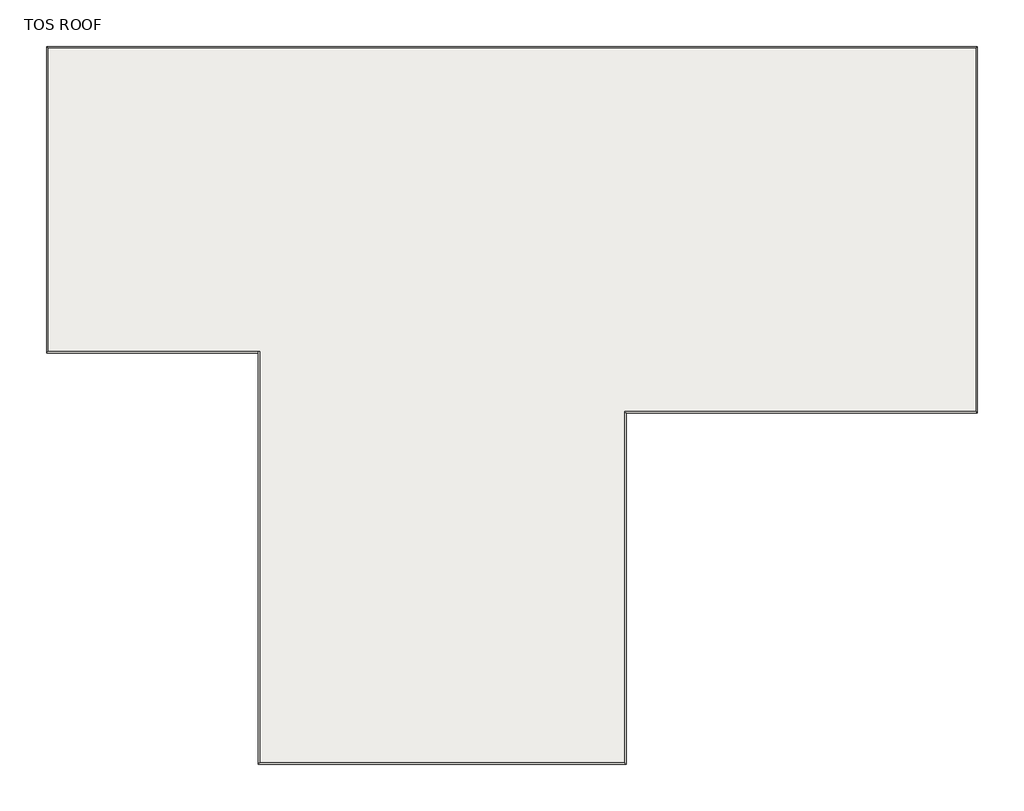
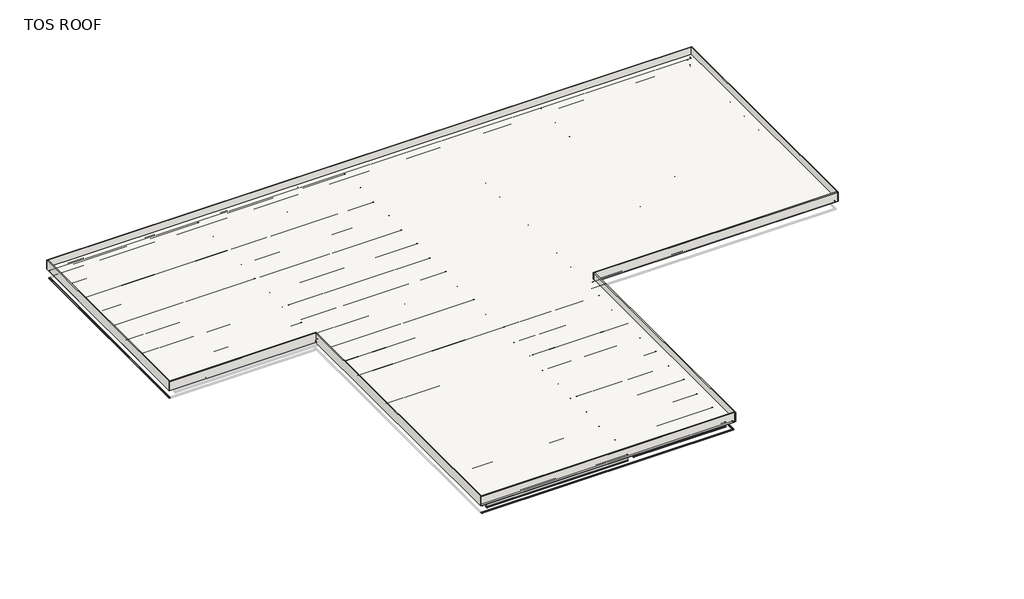
# One storey, part 1 of 3: 41 beams, 8 walls, 1 roof, 1 slab.
# Revit data of these elements (continued)
# Type "Steel Framing_H_KS : H_SB_AR_S02_H-300x150x6.5x9_SRG3"
#   Type Comments = "MAIN"
#   Type Mark = "SRG3"
#   H_SectionID = "H-300x150x6.5x9"
#   H_Ratio for Additional Steel Plate = 0.2
#   Width = 15.0 cm
#   Web Thickness = 0.65 cm
#   Web Fillet = 1.3 cm
#   Warping Constant = 107000.0 cm⁶
#   Torsional Moment of Inertia = 9.9539 cm⁴
#   Section Area = 46.78 cm²
#   Plastic Modulus weak axis = 105.0 cm³
#   Plastic Modulus strong axis = 542.0 cm³
#   Perimeter = 1.17 m²/m
#   Nominal Weight = 36.70 kgf/m
#   Moment of Inertia weak axis = 508.00 cm⁴
#   Moment of Inertia strong axis = 7210.00 cm⁴
#   Height = 30.0 cm
#   Flange Thickness = 0.9 cm
#   Elastic Modulus weak axis = 67.7 cm³
#   Elastic Modulus strong axis = 481.0 cm³
#   Centroid Vertical = 15.0 cm
#   Centroid Horizontal = 7.5 cm
#   Bolt Spacing = 8.89 cm
#   Length [instance default] = 1500 mm
#   Structural Material [instance default] = Steel, 45-345
#   Section Name Key = ""
#   Assembly Code = ""
# Type "Steel Framing_H_KS : H_SB_AR_S02_H-800x300x14x26_SRB1"
#   Type Comments = "MAIN"
#   Type Mark = "SRB1"
#   H_SectionID = "H-800x300x14x26"
#   H_Ratio for Additional Steel Plate = 0.2
#   Width = 30.0 cm
#   Web Thickness = 1.4 cm
#   Web Fillet = 2.8 cm
#   Warping Constant = 17500000.0 cm⁶
#   Torsional Moment of Inertia = 422.315 cm⁴
#   Section Area = 267.4 cm²
#   Plastic Modulus weak axis = 1220.0 cm³
#   Plastic Modulus strong axis = 8240.0 cm³
#   Perimeter = 2.72 m²/m
#   Nominal Weight = 210.00 kgf/m
#   Moment of Inertia weak axis = 11700.00 cm⁴
#   Moment of Inertia strong axis = 292000.00 cm⁴
#   Height = 80.0 cm
#   Flange Thickness = 2.6 cm
#   Elastic Modulus weak axis = 782.0 cm³
#   Elastic Modulus strong axis = 7290.0 cm³
#   Centroid Vertical = 40.0 cm
#   Centroid Horizontal = 15.0 cm
#   Bolt Spacing = 8.89 cm
#   Length [instance default] = 1500 mm
#   Structural Material [instance default] = Steel, 45-345
#   Section Name Key = ""
#   Assembly Code = ""
# Type "Steel Framing_H_KS : H_SB_AR_S02_H-600x200x11x17_SRB2"
#   Type Comments = "MAIN"
#   Type Mark = "SRB2"
#   H_SectionID = "H-600x200x11x17"
#   H_Ratio for Additional Steel Plate = 0.2
#   Width = 20.0 cm
#   Web Thickness = 1.1 cm
#   Web Fillet = 2.2 cm
#   Warping Constant = 1930000.0 cm⁶
#   Torsional Moment of Inertia = 91.3724 cm⁴
#   Section Area = 134.4 cm²
#   Plastic Modulus weak axis = 361.0 cm³
#   Plastic Modulus strong axis = 2980.0 cm³
#   Perimeter = 1.94 m²/m
#   Nominal Weight = 106.00 kgf/m
#   Moment of Inertia weak axis = 2280.00 cm⁴
#   Moment of Inertia strong axis = 77600.00 cm⁴
#   Height = 60.0 cm
#   Flange Thickness = 1.7 cm
#   Elastic Modulus weak axis = 228.0 cm³
#   Elastic Modulus strong axis = 2590.0 cm³
#   Centroid Vertical = 30.0 cm
#   Centroid Horizontal = 10.0 cm
#   Bolt Spacing = 8.89 cm
#   Length [instance default] = 1500 mm
#   Structural Material [instance default] = Steel, 45-345
#   Section Name Key = ""
#   Assembly Code = ""
# Type "Steel Framing_H_KS : H_SB_AR_S02_H-800x300x14x26_SRG1"
#   Type Comments = "MAIN"
#   Type Mark = "SRG1"
#   H_SectionID = "H-800x300x14x26"
#   H_Ratio for Additional Steel Plate = 0.2
#   Width = 30.0 cm
#   Web Thickness = 1.4 cm
#   Web Fillet = 2.8 cm
#   Warping Constant = 17500000.0 cm⁶
#   Torsional Moment of Inertia = 422.315 cm⁴
#   Section Area = 267.4 cm²
#   Plastic Modulus weak axis = 1220.0 cm³
#   Plastic Modulus strong axis = 8240.0 cm³
#   Perimeter = 2.72 m²/m
#   Nominal Weight = 210.00 kgf/m
#   Moment of Inertia weak axis = 11700.00 cm⁴
#   Moment of Inertia strong axis = 292000.00 cm⁴
#   Height = 80.0 cm
#   Flange Thickness = 2.6 cm
#   Elastic Modulus weak axis = 782.0 cm³
#   Elastic Modulus strong axis = 7290.0 cm³
#   Centroid Vertical = 40.0 cm
#   Centroid Horizontal = 15.0 cm
#   Bolt Spacing = 8.89 cm
#   Length [instance default] = 1500 mm
#   Structural Material [instance default] = Steel, 45-345
#   Section Name Key = ""
#   Assembly Code = ""
# Type "Steel Framing_H_KS : H_SB_AR_S02_H-600x200x11x17_SRG2"
#   Type Comments = "MAIN"
#   Type Mark = "SRG2"
#   H_SectionID = "H-600x200x11x17"
#   H_Ratio for Additional Steel Plate = 0.2
#   Width = 20.0 cm
#   Web Thickness = 1.1 cm
#   Web Fillet = 2.2 cm
#   Warping Constant = 1930000.0 cm⁶
#   Torsional Moment of Inertia = 91.3724 cm⁴
#   Section Area = 134.4 cm²
#   Plastic Modulus weak axis = 361.0 cm³
#   Plastic Modulus strong axis = 2980.0 cm³
#   Perimeter = 1.94 m²/m
#   Nominal Weight = 106.00 kgf/m
#   Moment of Inertia weak axis = 2280.00 cm⁴
#   Moment of Inertia strong axis = 77600.00 cm⁴
#   Height = 60.0 cm
#   Flange Thickness = 1.7 cm
#   Elastic Modulus weak axis = 228.0 cm³
#   Elastic Modulus strong axis = 2590.0 cm³
#   Centroid Vertical = 30.0 cm
#   Centroid Horizontal = 10.0 cm
#   Bolt Spacing = 8.89 cm
#   Length [instance default] = 1500 mm
#   Structural Material [instance default] = Steel, 45-345
#   Section Name Key = ""
#   Assembly Code = ""
# Type "Steel Framing_LC : H_SB_AR_S00_LC-150x75x25x3.2"
#   Type Comments = "SECONDARY"
#   Type Mark = "GIRTH"
#   H_SectionID = "LC-150x75x25x3.2"
#   r = 4.8 mm
#   d = 25 mm
#   R = 8 mm
#   Perimeter = 0.70 m²/m
#   Nominal Weight = 10.30 kgf/m
#   Length [instance default] = 1000 mm
#   b = 75 mm
#   h = 150 mm
#   tw = 3.2 mm
#   x = 18.6 mm
#   A = 1.00 m²
#   Structural Material [instance default] = Steel, 45-345
#   Assembly Code = ""
# Type "H_RF_AR_B06_Memb_XPS_PE_Protective Conc_SkyPanel Roof_T160"
#   Layers, outside or top first: 0 mm no material (function 100); 0 mm no material (function 100); 160 mm no material (function 3); 0 mm no material (function 100)
# Type "H_FL_AR_S17_RC Deck Slab_T150_RS1"
#   Keynote = ""
#   Type Comments = "AG"
#   Description = ""
#   Type Mark = "RS1"
#   H_Rebar Ratio = 0.1
#   Function = 1
#   Layers, outside or top first: 150 mm "00_Concrete_Reinf. Conc." (function 1); 0 mm no material (function 200)
# Type "H_WA_AR_B02_Ext Wall_RC_Parapet_Exposed_T120"
#   Type Comments = ""
#   Layers, outside or top first: 0 mm no material (function 100); 0 mm no material (function 100); 120 mm no material (function 1); 0 mm no material (function 100); 0 mm no material (function 100); 0 mm no material (function 100)
# Elements 1, 2, 3, 7, 8, 10, 11, 12, 13, 14, 15, 16, 17, 18, 19 (IfcBeam, "Steel Framing_H_KS : H_SB_AR_S02_H-300x150x6.5x9_SRG3")
#   Structural Material = Steel, 45-345
#   Phase Created = New Construction
#   Materials on its faces: "Steel, 45-345"
# Elements 4, 5, 6, 24, 25 (IfcBeam, "Steel Framing_H_KS : H_SB_AR_S02_H-800x300x14x26_SRB1")
#   Structural Material = Steel, 45-345
#   Phase Created = New Construction
#   Materials on its faces: "Steel, 45-345"
# Elements 9, 20, 21, 22, 23 (IfcBeam, "Steel Framing_H_KS : H_SB_AR_S02_H-600x200x11x17_SRB2")
#   Structural Material = Steel, 45-345
#   Phase Created = New Construction
#   Materials on its faces: "Steel, 45-345"
# Elements 26, 27, 28, 29, 30 (IfcBeam, "Steel Framing_H_KS : H_SB_AR_S02_H-800x300x14x26_SRG1")
#   Structural Material = Steel, 45-345
#   Phase Created = New Construction
#   Materials on its faces: "Steel, 45-345"
# Elements 31, 32, 33, 34, 35 (IfcBeam, "Steel Framing_H_KS : H_SB_AR_S02_H-600x200x11x17_SRG2")
#   Structural Material = Steel, 45-345
#   Phase Created = New Construction
#   Materials on its faces: "Steel, 45-345"
# Elements 36, 37, 38, 39, 40, 41 (IfcBeam, "Steel Framing_LC : H_SB_AR_S00_LC-150x75x25x3.2")
#   Structural Material = Steel, 45-345
#   Phase Created = New Construction
#   Materials on its faces: "Steel, 45-345"
# Element 42 (IfcRoof, "H_RF_AR_B06_Memb_XPS_PE_Protective Conc_SkyPanel Roof_T160")
#   built-in parameter 1001705 = 34.4815 (stored number, unit not read)
#   built-in parameter 1001701 = 0.492126 (stored number, unit not read)
#   built-in parameter 1001710 = 33615
#   Phase Created = New Construction
#   Materials on its faces: "Default Roof"
# Element 43 (IfcSlab, "H_FL_AR_S17_RC Deck Slab_T150_RS1")
#   Height Offset From Level = 150 mm
#   Phase Created = New Construction
#   Materials on its faces: "Default Floor", "00_Concrete_Reinf. Conc."
# Elements 44, 45, 46, 47, 48, 49, 50, 51 (IfcWall, "H_WA_AR_B02_Ext Wall_RC_Parapet_Exposed_T120")
#   Comments = ""
#   Top Offset = 0 mm
#   Base Offset = 0 mm
#   Unconnected Height = 1200 mm
#   wall height = 1200 mm
#   Phase Created = New Construction
#   Base Constraint = TOS ROOF
#   Materials on its faces: "Default Wall"
# Materials
#   "Steel, 45-345": class "Metal", colour RGB 189 187 185, transparency 0, Description = "Steel 345 MPa", Cost = 0
#   "00_Concrete_Reinf. Conc.": class "Concrete", colour RGB 176 176 176, transparency 0, Description = "Reinf. Conc.", Cost = 0, Image = Concrete.Cast-In-Place.Flat.Polished.Grey.jpg
#   "Default Roof": class "Miscellaneous", colour RGB 80 80 80, transparency 0
#   "Default Floor": class "Miscellaneous", colour RGB 80 80 80, transparency 0
#   "Default Wall": class "Miscellaneous", colour RGB 80 80 80, transparency 0, Description = "SANDWICH PANEL"
